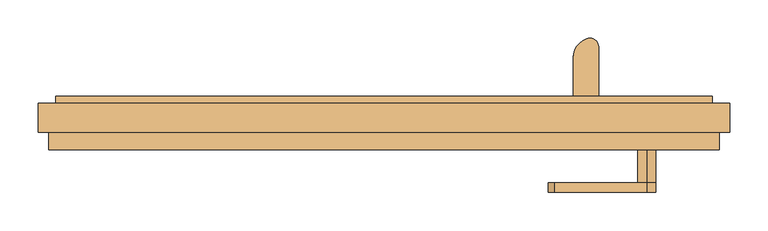
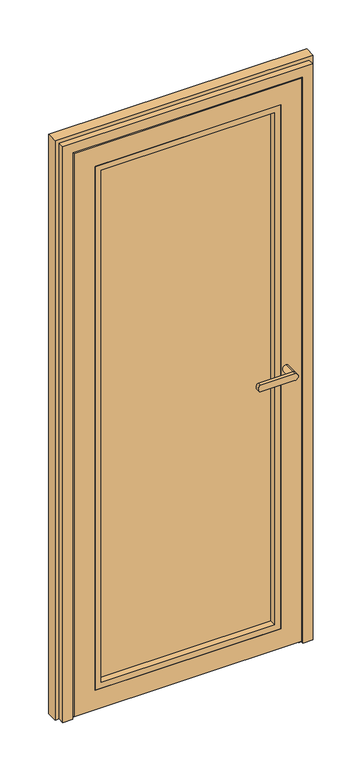
"""IFC4 building model written with IfcOpenShell, lengths in millimetres: door geometry, Schueco_FWS_ADS-70-HD_inw_Family-01 : FWS SI insert unit."""

from ifc_helpers import new_model, si_unit, point, frame, frame_2d, origin, place, context, project, spatial, polyline, circle_curve, ellipse_curve, trimmed, segment, composite_curve, outline, extrude, faceted_brep, source, transform, mapped, element, save
from ifc_brep_helpers import plane_surface, cylinder_surface, extruded_surface, advanced_brep


def door_d7f0f1dc(model_context):
    return source(origin(), model_context, "Body", "SolidModel", [
        extrude(outline(composite_curve([segment(polyline([(248.3337564, 8.9997177), (248.3337564, 59.1618682)]), True, "CONTINUOUS"), segment(trimmed(circle_curve(frame_2d((275.512174, 59.1618682)), 27.1784177), [point((248.3337564, 59.1618682))], [point((265.9750784, 84.6120194))], False, "CARTESIAN"), True, "CONTINUOUS"), segment(trimmed(circle_curve(frame_2d((270.0525794, 73.7310321)), 11.6198924), [point((265.9750784, 84.6120194))], [point((281.6724718, 73.7310321))], False, "CARTESIAN"), True, "CONTINUOUS"), segment(polyline([(281.6724718, 73.7310321), (281.6724718, 8.9997177), (248.3337564, 8.9997177)]), True, "CONTINUOUS")], self_intersect=False)), frame((0.0, 0.0, 2053.9218203), z_axis=(0.0, 0.0, 1.0), x_axis=(1.0, 0.0, 0.0)), (0.0, 0.0, 1.0), 4.0),
        extrude(outline(polyline([(248.3337564, 12.9997177), (281.6724718, 12.9997177), (281.6724718, 8.9997177), (248.3337564, 8.9997177), (248.3337564, 12.9997177)])), frame((0.0, 0.0, 2023.9218203), z_axis=(0.0, 0.0, 1.0), x_axis=(1.0, 0.0, 0.0)), (0.0, 0.0, 1.0), 30.0),
        extrude(outline(polyline([(248.3337564, 12.9997177), (281.6724718, 12.9997177), (281.6724718, 8.9997177), (248.3337564, 8.9997177), (248.3337564, 12.9997177)])), frame((0.0, 0.0, 49.9218203), z_axis=(0.0, 0.0, 1.0), x_axis=(1.0, 0.0, 0.0)), (0.0, 0.0, 1.0), 30.0),
        extrude(outline(composite_curve([segment(polyline([(248.3337564, 8.9997177), (248.3337564, 59.1618682)]), True, "CONTINUOUS"), segment(trimmed(circle_curve(frame_2d((275.512174, 59.1618682)), 27.1784177), [point((248.3337564, 59.1618682))], [point((265.9750784, 84.6120194))], False, "CARTESIAN"), True, "CONTINUOUS"), segment(trimmed(circle_curve(frame_2d((270.0525794, 73.7310321)), 11.6198924), [point((265.9750784, 84.6120194))], [point((281.6724718, 73.7310321))], False, "CARTESIAN"), True, "CONTINUOUS"), segment(polyline([(281.6724718, 73.7310321), (281.6724718, 8.9997177), (248.3337564, 8.9997177)]), True, "CONTINUOUS")], self_intersect=False)), frame((0.0, 0.0, 45.9218203), z_axis=(0.0, 0.0, 1.0), x_axis=(1.0, 0.0, 0.0)), (0.0, 0.0, 1.0), 4.0),
        advanced_brep(
        [(277.718156, 57.5977179, 2053.9218203), (252.2840039, 72.2821425, 2053.9218203), (277.718156, 57.5977179, 49.9218203), (252.2840039, 72.2821425, 49.9218203)],
        [
            (0, 1, ellipse_curve(frame((265.0010799, 64.9399302, 2053.9218203), z_axis=(0.0, 0.0, 1.0000000000000002), x_axis=(0.5000002582658958, 0.866025254674503, 0.0)), 21.5840887, 14.6844171)),
            (1, 0, ellipse_curve(frame((265.0010799, 64.9399302, 2053.9218203), z_axis=(0.0, 0.0, 1.0000000000000002), x_axis=(0.5000002582658958, 0.866025254674503, 0.0)), 21.5840887, 14.6844171)),
            (2, 3, ellipse_curve(frame((265.0010799, 64.9399302, 49.9218203), z_axis=(0.0, 0.0, -1.0000000000000002), x_axis=(-0.866025254674503, 0.5000002582658958, 0.0)), 14.6844171, 21.5840887)),
            (3, 2, ellipse_curve(frame((265.0010799, 64.9399302, 49.9218203), z_axis=(0.0, 0.0, -1.0000000000000002), x_axis=(-0.866025254674503, 0.5000002582658958, 0.0)), 14.6844171, 21.5840887)),
            (0, 2),
            (3, 1),
        ],
        [
            plane_surface(frame((252.2840039, 72.2821425, 2053.9218203), z_axis=(0.0, 0.0, 1.0000000000000002), x_axis=(0.5000002582658958, 0.866025254674503, 0.0))),
            plane_surface(frame((252.2840039, 72.2821425, 49.9218203), z_axis=(0.0, 0.0, -1.0000000000000002), x_axis=(-0.5000002582658958, -0.866025254674503, 0.0))),
            extruded_surface(trimmed(ellipse_curve(frame((265.0010799, 64.9399302, 49.9218203), z_axis=(0.0, 0.0, -1.0000000000000002), x_axis=(-0.866025254674503, 0.5000002582658958, 0.0)), 14.6844171, 21.5840887), [point((252.2840039, 72.2821425, 49.9218203))], [point((277.718156, 57.5977179, 49.9218203))], True, "CARTESIAN"), (0.0, 0.0, -2004.0), 2004.0),
            extruded_surface(trimmed(ellipse_curve(frame((265.0010799, 64.9399302, 49.9218203), z_axis=(0.0, 0.0, -1.0000000000000002), x_axis=(-0.866025254674503, 0.5000002582658958, 0.0)), 14.6844171, 21.5840887), [point((277.718156, 57.5977179, 49.9218203))], [point((252.2840039, 72.2821425, 49.9218203))], True, "CARTESIAN"), (0.0, 0.0, -2004.0), 2004.0),
        ],
        [
            (0, [[1, 2]]),
            (1, [[3, 4]]),
            (2, [[5, -4, 6, -1]]),
            (3, [[-6, -3, -5, -2]]),
        ],
    ),
        advanced_brep(
        [(345.0010799, -117.0002518, 1030.9991882), (345.0010799, -117.0002518, 1054.9764498), (223.3392873, -117.0002518, 1054.9764498), (223.3392873, -117.0002518, 1030.9991882), (345.0010799, -104.5001648, 1054.9764498), (345.0010799, -104.5001648, 1030.9991882), (223.3392873, -104.5001648, 1030.9991882), (223.3392873, -104.5001648, 1054.9764498), (345.0010799, -61.0002823, 1030.9991882), (345.0010799, -61.0002823, 1054.9764498)],
        [
            (0, 1, circle_curve(frame((345.0010799, -117.0002518, 1042.987819), z_axis=(0.0, -1.0, 0.0), x_axis=(0.0, 0.0, 1.0)), 11.9886308)),
            (1, 2),
            (2, 3, ellipse_curve(frame((223.3392873, -117.0002518, 1042.987819), z_axis=(0.0, -1.0, 0.0), x_axis=(0.0, 0.0, -1.0)), 11.9886308, 7.9050795)),
            (3, 0),
            (4, 5, circle_curve(frame((345.0010799, -104.5001648, 1042.987819), z_axis=(0.0, -1.0, 0.0), x_axis=(0.0, 0.0, 1.0)), 11.9886308)),
            (5, 6),
            (6, 7, ellipse_curve(frame((223.3392873, -104.5001648, 1042.987819), z_axis=(0.0, 1.0, 0.0), x_axis=(0.0, 0.0, -1.0)), 11.9886308, 7.9050795)),
            (7, 4),
            (3, 6),
            (5, 0),
            (2, 7),
            (1, 4),
            (5, 4, circle_curve(frame((345.0010799, -104.5001648, 1042.987819), z_axis=(0.0, -1.0, 0.0), x_axis=(0.0, 0.0, 1.0)), 11.9886308)),
            (8, 9, circle_curve(frame((345.0010799, -61.0002823, 1042.987819), z_axis=(0.0, 1.0, 0.0), x_axis=(0.0, 0.0, 1.0)), 11.9886308)),
            (9, 8, circle_curve(frame((345.0010799, -61.0002823, 1042.987819), z_axis=(0.0, 1.0, 0.0), x_axis=(0.0, 0.0, 1.0)), 11.9886308)),
            (8, 5),
            (4, 9),
        ],
        [
            plane_surface(frame((223.3392873, -117.0002518, 1030.9991882), z_axis=(0.0, -1.0, 0.0), x_axis=(-1.0, 0.0, 0.0))),
            plane_surface(frame((223.3392873, -104.5001648, 1030.9991882), z_axis=(0.0, 1.0, 0.0), x_axis=(1.0, 0.0, 0.0))),
            plane_surface(frame((345.0010799, -117.0002518, 1030.9991882), z_axis=(0.0, 0.0, -1.0), x_axis=(0.0, 1.0, 0.0))),
            extruded_surface(trimmed(ellipse_curve(frame((223.3392873, -104.5001648, 1042.987819), z_axis=(0.0, 1.0, 0.0), x_axis=(0.0, 0.0, -1.0)), 11.9886308, 7.9050795), [point((223.3392873, -104.5001648, 1030.9991882))], [point((223.3392873, -104.5001648, 1054.9764498))], True, "CARTESIAN"), (0.0, 12.500086999999994, 0.0), 12.500086999999994),
            plane_surface(frame((223.3392873, -117.0002518, 1054.9764498), z_axis=(0.0, 0.0, 1.0), x_axis=(0.0, 1.0, 0.0))),
            cylinder_surface(frame((345.0010799, -104.5001648, 1042.987819), z_axis=(0.0, -1.0, 0.0), x_axis=(0.0, 0.0, 1.0)), 11.9886308),
            plane_surface(frame((345.0010799, -61.0002823, 1054.9764498), z_axis=(0.0, 1.0, 0.0), x_axis=(-1.0, 0.0, 0.0))),
            cylinder_surface(frame((345.0010799, -61.0002823, 1042.987819), z_axis=(0.0, -1.0, 0.0), x_axis=(0.0, 0.0, 1.0)), 11.9886308),
        ],
        [
            (0, [[1, 2, 3, 4]]),
            (1, [[5, 6, 7, 8]]),
            (2, [[9, -6, 10, -4]]),
            (3, [[11, -7, -9, -3]]),
            (4, [[12, -8, -11, -2]]),
            (5, [[-10, 13, -12, -1]]),
            (6, [[14, 15]]),
            (7, [[16, -5, 17, -14]]),
            (7, [[-17, -13, -16, -15]]),
        ],
    ),
        extrude(outline(polyline([(80.9218203, 327.0670787), (2027.0538178, 327.0670787), (2027.0538178, -327.0649188), (80.9218203, -327.0649188), (80.9218203, 327.0670787)]), holes=[polyline([(102.9234681, -305.063271), (2005.05217, -305.063271), (2005.05217, 305.0654309), (102.9234681, 305.0654309), (102.9234681, -305.063271)])]), frame((0.0, -61.0002823, 0.0), z_axis=(0.0, 1.0, 0.0), x_axis=(0.0, 0.0, 1.0)), (0.0, 0.0, 1.0), 23.0002823),
        faceted_brep([(-399.9989201, -61.0002823, 2099.987819), (-399.9989201, -52.5000065, 2099.987819), (-399.9989201, -52.5000065, 7.987819), (-399.9989201, -61.0002823, 7.987819), (400.0010799, -52.5000065, 7.987819), (400.0010799, -61.0002823, 7.987819), (400.0010799, -52.5000065, 2099.987819), (385.0670787, -52.5000065, 22.9218203), (385.0670787, -52.5000065, 2085.0538178), (-385.0649188, -52.5000065, 2085.0538178), (-385.0649188, -52.5000065, 22.9218203), (400.0010799, -61.0002823, 2099.987819), (-327.0649188, -61.0002823, 80.9218203), (-327.0649188, -61.0002823, 2027.0538178), (327.0670787, -61.0002823, 2027.0538178), (327.0670787, -61.0002823, 80.9218203), (-327.0649188, 0.0, 2027.0538178), (-327.0649188, 0.0, 80.9218203), (327.0670787, 0.0, 80.9218203), (327.0670787, 0.0, 2027.0538178), (-302.0649188, 0.0, 105.9218203), (-302.0649188, 0.0, 2002.0538178), (302.0670787, 0.0, 2002.0538178), (302.0670787, 0.0, 105.9218203), (-302.0649188, 8.9997177, 2002.0538178), (-302.0649188, 8.9997177, 105.9218203), (302.0670787, 8.9997177, 105.9218203), (302.0670787, 8.9997177, 2002.0538178), (-375.0649188, 8.9997177, 32.9218203), (-375.0649188, 8.9997177, 2075.0538178), (375.0670787, 8.9997177, 2075.0538178), (375.0670787, 8.9997177, 32.9218203), (-375.0649188, 0.4997603, 2075.0538178), (-375.0649188, 0.4997603, 32.9218203), (375.0670787, 0.4997603, 32.9218203), (375.0670787, 0.4997603, 2075.0538178), (-385.0649188, 0.4997603, 22.9218203), (-385.0649188, 0.4997603, 2085.0538178), (385.0670787, 0.4997603, 2085.0538178), (385.0670787, 0.4997603, 22.9218203)], [[[0, 1, 2, 3]], [[3, 2, 4, 5]], [[2, 1, 6, 4], [7, 8, 9, 10]], [[5, 4, 6, 11]], [[5, 11, 0, 3], [12, 13, 14, 15]], [[16, 13, 12, 17]], [[17, 12, 15, 18]], [[18, 15, 14, 19]], [[18, 19, 16, 17], [20, 21, 22, 23]], [[24, 21, 20, 25]], [[25, 20, 23, 26]], [[26, 23, 22, 27]], [[28, 29, 30, 31], [26, 27, 24, 25]], [[32, 29, 28, 33]], [[33, 28, 31, 34]], [[34, 31, 30, 35]], [[36, 37, 38, 39], [34, 35, 32, 33]], [[9, 37, 36, 10]], [[10, 36, 39, 7]], [[7, 39, 38, 8]], [[11, 6, 1, 0]], [[19, 14, 13, 16]], [[27, 22, 21, 24]], [[35, 30, 29, 32]], [[8, 38, 37, 9]]]),
        extrude(outline(polyline([(327.0670787, -38.0), (-327.0649188, -38.0), (-327.0649188, 0.0), (327.0670787, 0.0), (327.0670787, -38.0)])), frame((0.0, 0.0, 80.9218203), z_axis=(0.0, 0.0, 1.0), x_axis=(1.0, 0.0, 0.0)), (0.0, 0.0, 1.0), 1946.1319975),
        extrude(outline(composite_curve([segment(trimmed(circle_curve(frame_2d((-36.8963068, 15.7489666)), 15.8153344), [point((-26.2439405, 4.0591464))], [point((-47.548673, 4.0591464))], False, "CARTESIAN"), True, "CONTINUOUS"), segment(polyline([(-47.548673, 4.0591464), (-47.548673, 22.9218203), (-26.2439405, 22.9218203), (-26.2439405, 4.0591464)]), True, "CONTINUOUS")], self_intersect=False)), frame((-385.0649188, 0.0, 0.0), z_axis=(1.0, 0.0, 0.0), x_axis=(0.0, 1.0, 0.0)), (0.0, 0.0, 1.0), 770.1319975),
        extrude(outline(polyline([(-375.0649188, 0.4997603), (-375.0649188, 8.9997177), (375.0670787, 8.9997177), (375.0670787, 0.4997603), (-375.0649188, 0.4997603)])), frame((0.0, 0.0, 7.9218203), z_axis=(0.0, 0.0, 1.0), x_axis=(1.0, 0.0, 0.0)), (0.0, 0.0, 1.0), 25.0),
        faceted_brep([(430.999943, 8.9997177, 2130.999943), (430.999943, 0.0, 2130.999943), (430.999943, 0.0, 0.0), (430.999943, 8.9997177, 0.0), (-454.0, 0.0, 0.0), (-454.0, 0.0, 2154.0), (454.0, 0.0, 2154.0), (454.0, 0.0, 0.0), (-430.999943, 0.0, 2130.999943), (-430.999943, 0.0, 0.0), (454.0, -38.0, 0.0), (440.0, -38.0, 0.0), (440.0, -61.0002823, 0.0), (404.9999411, -61.0002823, 0.0), (404.9999411, -52.5000065, 0.0), (394.9999487, -52.5000065, 0.0), (394.9999487, 0.4997603, 0.0), (379.9999888, 0.4997603, 0.0), (379.9999888, 8.9997177, 0.0), (-379.9999888, 8.9997177, 0.0), (-430.999943, 8.9997177, 0.0), (-430.999943, 8.9997177, 2130.999943), (379.9999888, 8.9997177, 2079.9999888), (-379.9999888, 8.9997177, 2079.9999888), (404.9999411, -61.0002823, 2104.9999411), (404.9999411, -52.5000065, 2104.9999411), (-404.9999411, -52.5000065, 0.0), (-394.9999487, -52.5000065, 0.0), (-394.9999487, -52.5000065, 2094.9999487), (394.9999487, -52.5000065, 2094.9999487), (-404.9999411, -52.5000065, 2104.9999411), (-440.0, -61.0002823, 0.0), (-404.9999411, -61.0002823, 0.0), (-404.9999411, -61.0002823, 2104.9999411), (440.0, -61.0002823, 2140.0), (-440.0, -61.0002823, 2140.0), (440.0, -38.0, 2140.0), (-454.0, -38.0, 0.0), (-440.0, -38.0, 0.0), (-440.0, -38.0, 2140.0), (454.0, -38.0, 2154.0), (-454.0, -38.0, 2154.0), (-379.9999888, 0.4997603, 0.0), (-394.9999487, 0.4997603, 0.0), (379.9999888, 0.4997603, 2079.9999888), (-379.9999888, 0.4997603, 2079.9999888), (394.9999487, 0.4997603, 2094.9999487), (-394.9999487, 0.4997603, 2094.9999487)], [[[0, 1, 2, 3]], [[4, 5, 6, 7, 2, 1, 8, 9]], [[3, 2, 7, 10, 11, 12, 13, 14, 15, 16, 17, 18]], [[19, 20, 21, 0, 3, 18, 22, 23]], [[24, 25, 14, 13]], [[26, 27, 28, 29, 15, 14, 25, 30]], [[31, 32, 33, 24, 13, 12, 34, 35]], [[34, 12, 11, 36]], [[37, 38, 39, 36, 11, 10, 40, 41]], [[4, 9, 20, 19, 42, 43, 27, 26, 32, 31, 38, 37]], [[20, 9, 8, 21]], [[18, 17, 44, 22]], [[42, 19, 23, 45]], [[32, 26, 30, 33]], [[31, 35, 39, 38]], [[4, 37, 41, 5]], [[6, 40, 10, 7]], [[43, 42, 45, 44, 17, 16, 46, 47]], [[16, 15, 29, 46]], [[27, 43, 47, 28]], [[21, 8, 1, 0]], [[33, 30, 25, 24]], [[35, 34, 36, 39]], [[23, 22, 44, 45]], [[5, 41, 40, 6]], [[47, 46, 29, 28]]]),
    ])


if __name__ == "__main__":
    model = new_model("IFC4")
    model_context = context("Model", 3, world=origin())
    ifc_project = project(units=[si_unit("LENGTHUNIT", "METRE", prefix="MILLI")], contexts=[model_context])
    site = spatial("IfcSite", under=ifc_project)
    building = spatial("IfcBuilding", under=site)
    placement = place(None, origin())
    door_shape = door_d7f0f1dc(model_context)
    element("IfcDoor", 1, ObjectType="Schueco_FWS_ADS-70-HD_inw_Family-01 : FWS SI insert unit", at=placement, inside=building, context=model_context, shape_type="MappedRepresentation", body=[
        mapped(door_shape, transform((0.0, 0.0, 0.0), x_axis=(1.0, 0.0, 0.0), y_axis=(0.0, 1.0, 0.0), z_axis=(0.0, 0.0, 1.0))),
    ])
    save(model, "model.ifc")

# Revit data of these elements
# Type "Schueco_FWS_ADS-70-HD_inw_Family-01 : FWS SI insert unit"
#   Type Mark = "40"
#   __NOTE__ = "Data describes the optimum values of the entire system. The properites of a selected design option have to be determined on an individual basis!"
#   Wind load resistance = "Class 2"
#   Watertightness = "Class 5A"
#   Thermal insulation = "Uf = 1.6 W/(m²K)"
#   Sound insulation = "to RW 43 db"
#   Schueco thermal insulation standard = "Thermally insulated"
#   Opening type = "Inward-opening, Flush-fitted"
#   Model = "Schueco ADS 70 HD"
#   Mechanical loading = "Class 2"
#   Maximum leaf width in mm = "1400"
#   Maximum leaf weight in kg = "200"
#   Maximum leaf height in mm = "3000"
#   Material = "Aluminium"
#   Construction Type = "Door, single-leaf, inward-opening"
#   Manufacturer = "Schueco International KG"
#   Long term functionality = "Class 6"
#   Glazing data = "Triple glazing 38mm"
#   Façade insert unit = "yes"
#   Family creation date = "08.2017"
#   Description = "Schueco Aluminium Door System (ADS)"
#   Burglar resistance = "Class RC 3"
#   Areas of use = "Public buildings"
#   Analytic Construction = "<None>"
#   Air permeability = "Class 2"
#   Width [instance default] = 946.941 mm
#   Leaf opening angle [instance default] = 0.00°
#   IOf_T = 38 mm
#   Height [instance default] = 1988.68 mm
#   Glazing area [instance default] = 1.11272 m²
#   Distance from bottom to handles [instance default] = 1050 mm
#   Clear opening width [instance default] = 798.941 mm
#   Standard threshold = no
#   Low level threshold = yes
#   Handles = yes
#   FWS SI insert unit = yes
#   FWS HI insert unit = no
#   Glass = none
#   Frame = Alu
#   Fittings = none
# Element 1 (IfcDoor, "Schueco_FWS_ADS-70-HD_inw_Family-01 : FWS SI insert unit")
#   Width = 908 mm
#   Height = 2154 mm
#   Glazing area = 1.14518 m²
#   Clear opening width = 760 mm
#   Materials on its faces: "Alu", "Glass"
# Materials
#   "Alu": class "Glas", colour RGB 140 140 140, transparency 0
#   "Glass": class "Glass", colour RGB 128 128 255, transparency 0.75, Description = "Soda Lime Glass", Cost = 0
